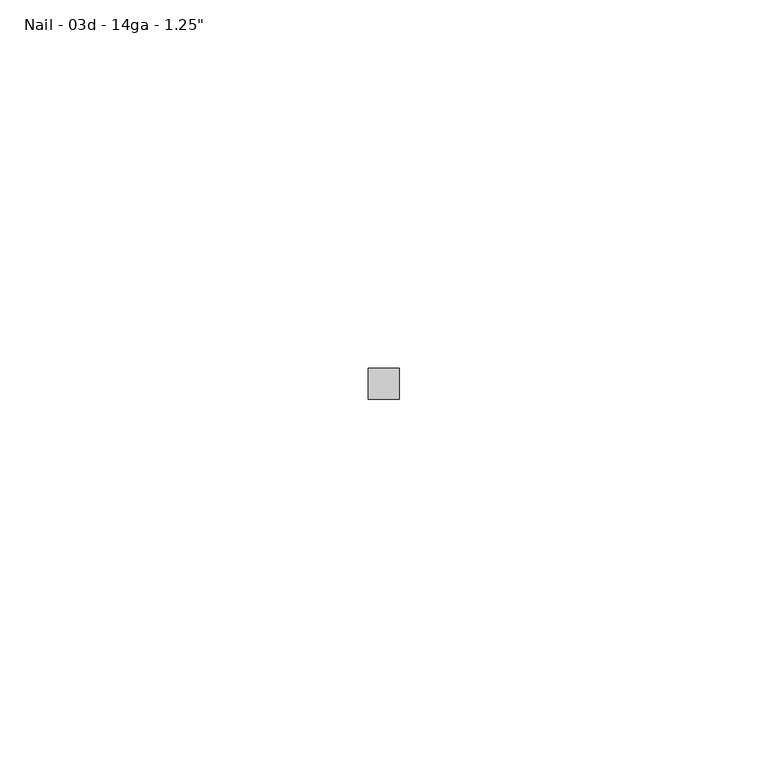
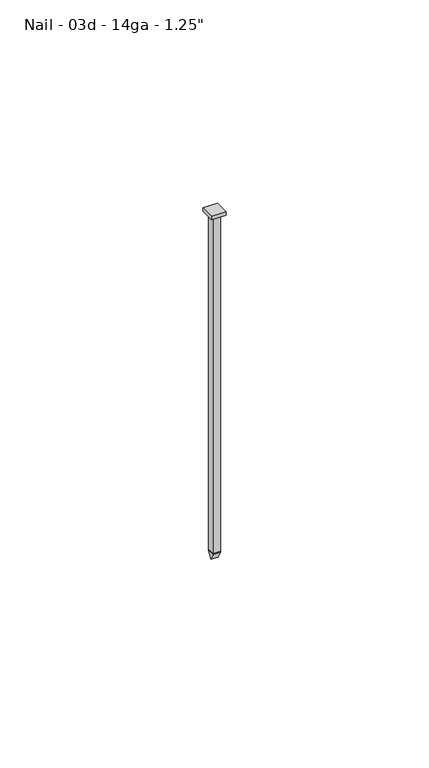
"""IFC4 building model written with IfcOpenShell, lengths in millimetres: fastener geometry."""

from ifc_helpers import new_model, si_unit, frame, origin, origin_with_axes, place, context, project, spatial, polyline, outline, extrude, source, transform, mapped, element, save


def fastener_3689d9c7(model_context):
    return source(origin(), model_context, "Body", "SweptSolid", [
        extrude(outline(polyline([(0.0, -103.7082), (-1.0541, -101.6), (1.0541, -101.6), (0.0, -103.7082)])), frame((-1.0541, 0.0, 0.0), z_axis=(1.0, 0.0, 0.0), x_axis=(0.0, 1.0, 0.0)), (0.0, 0.0, 1.0), 2.1082),
        extrude(outline(polyline([(-2.1082, -2.1082), (-2.1082, 2.1082), (2.1082, 2.1082), (2.1082, -2.1082), (-2.1082, -2.1082)])), origin_with_axes(), (0.0, 0.0, 1.0), 1.0541),
        extrude(outline(polyline([(-1.0541, 1.0541), (1.0541, 1.0541), (1.0541, -1.0541), (-1.0541, -1.0541), (-1.0541, 1.0541)])), frame((0.0, 0.0, -101.6), z_axis=(0.0, 0.0, 1.0), x_axis=(1.0, 0.0, 0.0)), (0.0, 0.0, 1.0), 101.6),
    ])


if __name__ == "__main__":
    model = new_model("IFC4")
    model_context = context("Model", 3, world=origin())
    ifc_project = project(units=[si_unit("LENGTHUNIT", "METRE", prefix="MILLI")], contexts=[model_context])
    site = spatial("IfcSite", under=ifc_project)
    building = spatial("IfcBuilding", under=site)
    placement = place(None, origin())
    fastener_shape = fastener_3689d9c7(model_context)
    element("IfcFastener", 1, ObjectType="060523 - W_P_C - Fastenings - Generic - SQUARE : Nail - 03d - 14ga - 1.25\"", at=placement, inside=building, context=model_context, shape_type="MappedRepresentation", body=[
        mapped(fastener_shape, transform((0.0, 0.0, 0.0), x_axis=(1.0, 0.0, 0.0), y_axis=(0.0, 1.0, 0.0), z_axis=(0.0, 0.0, 1.0))),
    ])
    save(model, "model.ifc")

# Revit data of these elements
# Type "060523 - W_P_C - Fastenings - Generic - SQUARE : Nail - 03d - 14ga - 1.25\""
#   Washer_Thickness = 0' - 0.00333"
#   Washer Radius = 0' - 0.0515"
#   Washer Offset - Head = 0' - 0"
#   Washer Offset = 0' - 0"
#   Thickness_of_Substrate [instance default] = 0' - 1"
#   Side = 0' - 0 37/64"
#   Radius = 0' - 0.0415"
#   Length [instance default] = 0' - 1 1/4"
#   Head Size = 0' - 1"
#   Head Radius = 0' - 0 1/2"
#   Head Height = 0' - 0.01"
#   Double Diameter = 0' - 0.166"
#   Diameter = 0' - 0.083"
#   Default Elevation = 4' - 0"
#   Washer_Nut_Visibility = no
#   Washer_Head_Visibility = no
#   Round_Head_Visibility = yes
#   Point Visibility = yes
#   Nut_Visibility = no
#   Hex_Head_Visiblilty = no
#   Washer Material = none
#   Bolt Material (Size) = AT SILL - FASTENER AT 24" O.C.
# Element 1 (IfcFastener, "060523 - W_P_C - Fastenings - Generic - SQUARE : Nail - 03d - 14ga - 1.25\"")
#   Length = 0' - 4"
# Materials
#   "AT SILL - FASTENER AT 24\" O.C.": class "Generic", colour RGB 120 120 120, transparency 0, Cost = 0
